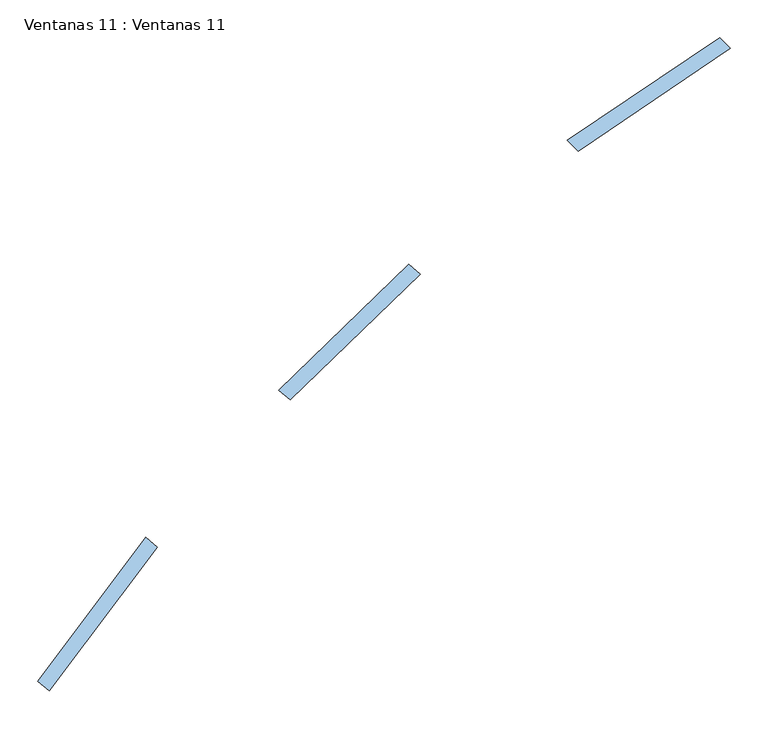
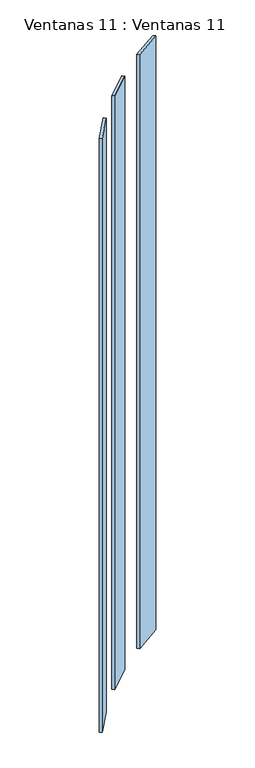
"""IFC4 building model written with IfcOpenShell, lengths in millimetres: window geometry, Ventanas 11 : Ventanas 11."""

from ifc_helpers import new_model, si_unit, frame, origin, place, context, project, spatial, polyline, outline, extrude, source, transform, mapped, element, save


def ventanas_11_ventanas_11_271d98a6(model_context):
    return source(origin(), model_context, "Body", "SweptSolid", [
        extrude(outline(polyline([(-8790.982532, -1005.1270266), (-8775.6616432, -1017.9827788), (-8919.745089, -1209.1879695), (-8935.0659779, -1196.3322173), (-8790.982532, -1005.1270266)])), frame((0.0, 0.0, 6206.6549752), z_axis=(0.0, 0.0, 1.0), x_axis=(1.0, 0.0, 0.0)), (0.0, 0.0, 1.0), 4832.8895714),
        extrude(outline(polyline([(-8441.5964303, -642.1563928), (-8426.2755415, -655.012145), (-8599.2074796, -822.0105764), (-8614.5283684, -809.1548242), (-8441.5964303, -642.1563928)])), frame((0.0, 0.0, 6206.6549752), z_axis=(0.0, 0.0, 1.0), x_axis=(1.0, 0.0, 0.0)), (0.0, 0.0, 1.0), 4832.8895714),
        extrude(outline(polyline([(-8027.6165959, -340.3628775), (-8013.4744602, -354.5050132), (-8216.16752, -491.2232083), (-8230.3096557, -477.0810727), (-8027.6165959, -340.3628775)])), frame((0.0, 0.0, 6206.6549752), z_axis=(0.0, 0.0, 1.0), x_axis=(1.0, 0.0, 0.0)), (0.0, 0.0, 1.0), 4832.8895714),
    ])


if __name__ == "__main__":
    model = new_model("IFC4")
    model_context = context("Model", 3, world=origin())
    ifc_project = project(units=[si_unit("LENGTHUNIT", "METRE", prefix="MILLI")], contexts=[model_context])
    site = spatial("IfcSite", under=ifc_project)
    building = spatial("IfcBuilding", under=site)
    placement = place(None, origin())
    ventanas_11_ventanas_11_shape = ventanas_11_ventanas_11_271d98a6(model_context)
    element("IfcWindow", 1, ObjectType="Ventanas 11 : Ventanas 11", at=placement, inside=building, context=model_context, shape_type="MappedRepresentation", body=[
        mapped(ventanas_11_ventanas_11_shape, transform((0.0, 0.0, 0.0), x_axis=(1.0, 0.0, 0.0), y_axis=(0.0, 1.0, 0.0), z_axis=(0.0, 0.0, 1.0))),
    ])
    save(model, "model.ifc")

# Revit data of these elements
# Type "Ventanas 11 : Ventanas 11"
#   Type Mark = "37"
# Element 1 (IfcWindow, "Ventanas 11 : Ventanas 11")
#   Materials on its faces: "VIDRIO"
# Materials
#   "VIDRIO": class "Genérico", colour RGB 120 120 120, transparency 0, Cost = 0
